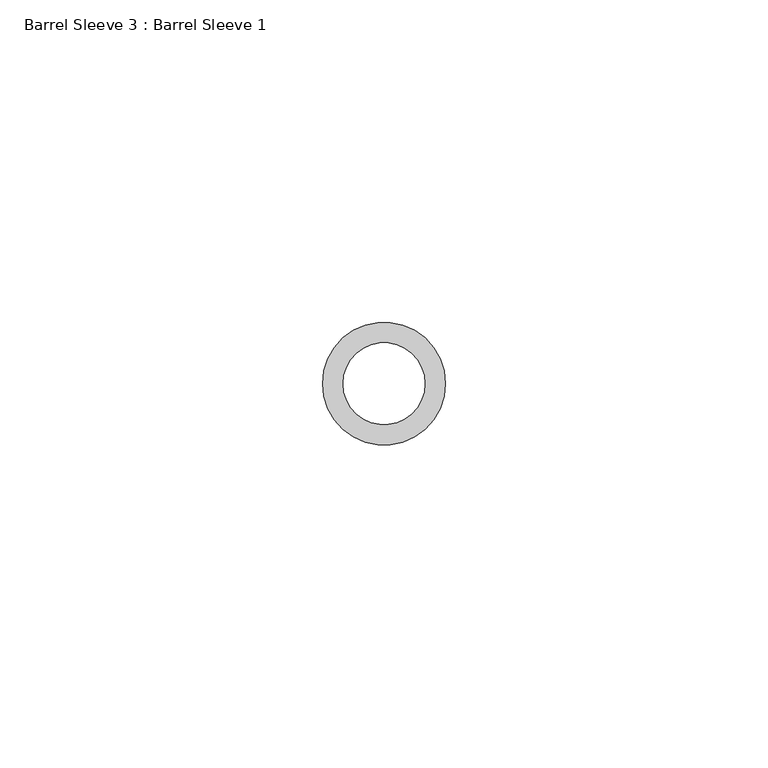
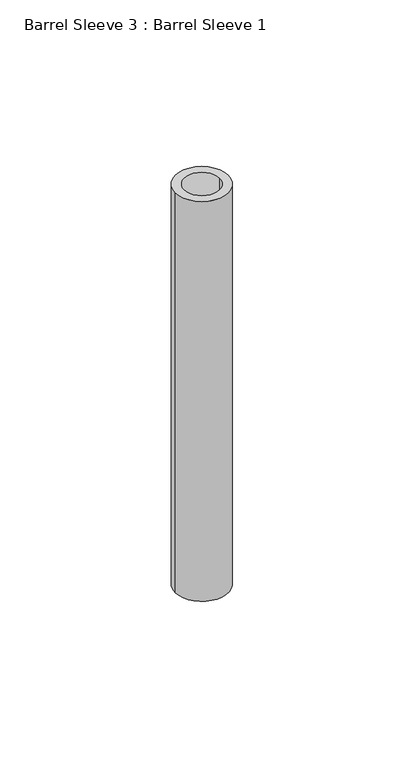
"""IFC4 building model written with IfcOpenShell, lengths in millimetres: proxy geometry, Barrel Sleeve 3 : Barrel Sleeve 1."""

from ifc_helpers import new_model, si_unit, point, frame, frame_2d, origin, place, context, project, spatial, circle_curve, trimmed, segment, composite_curve, outline, extrude, source, transform, mapped, element, save


def barrel_sleeve_3_barrel_sleeve_1_ca58ef70(model_context):
    return source(origin(), model_context, "Body", "SweptSolid", [
        extrude(outline(composite_curve([segment(trimmed(circle_curve(frame_2d((587309.5435739, -532839.3663841)), 9.525), [point((587300.0185739, -532839.3663841))], [point((587319.068574, -532839.3663841))], False, "CARTESIAN"), True, "CONTINUOUS"), segment(trimmed(circle_curve(frame_2d((587309.5435739, -532839.3663841)), 9.525), [point((587319.068574, -532839.3663841))], [point((587300.0185739, -532839.3663841))], False, "CARTESIAN"), True, "CONTINUOUS")], self_intersect=False), holes=[composite_curve([segment(trimmed(circle_curve(frame_2d((587309.5435739, -532839.3663841)), 6.35), [point((587303.1935739, -532839.3663841))], [point((587315.893574, -532839.3663841))], True, "CARTESIAN"), True, "CONTINUOUS"), segment(trimmed(circle_curve(frame_2d((587309.5435739, -532839.3663841)), 6.35), [point((587315.893574, -532839.3663841))], [point((587303.1935739, -532839.3663841))], True, "CARTESIAN"), True, "CONTINUOUS")], self_intersect=False)]), frame((0.0, 0.0, -152.4), z_axis=(0.0, 0.0, 1.0), x_axis=(1.0, 0.0, 0.0)), (0.0, 0.0, 1.0), 152.4),
    ])


if __name__ == "__main__":
    model = new_model("IFC4")
    model_context = context("Model", 3, world=origin())
    ifc_project = project(units=[si_unit("LENGTHUNIT", "METRE", prefix="MILLI")], contexts=[model_context])
    site = spatial("IfcSite", under=ifc_project)
    building = spatial("IfcBuilding", under=site)
    placement = place(None, origin())
    barrel_sleeve_3_barrel_sleeve_1_shape = barrel_sleeve_3_barrel_sleeve_1_ca58ef70(model_context)
    element("IfcBuildingElementProxy", 1, Name="Barrel Sleeve 3 : Barrel Sleeve 1", ObjectType="Barrel Sleeve 3 : Barrel Sleeve 1", at=placement, inside=building, context=model_context, shape_type="MappedRepresentation", body=[
        mapped(barrel_sleeve_3_barrel_sleeve_1_shape, transform((0.0, 0.0, 0.0), x_axis=(1.0, 0.0, 0.0), y_axis=(0.0, 1.0, 0.0), z_axis=(0.0, 0.0, 1.0))),
    ])
    save(model, "model.ifc")

# Revit data of these elements
# Element 1 (IfcBuildingElementProxy, "Barrel Sleeve 3 : Barrel Sleeve 1")
#   Materials on its faces: "5/8\" ID STEEL SLEEVE"
# Materials
#   "5/8\" ID STEEL SLEEVE": class "Metal", colour RGB 189 187 185, transparency 0, Description = "Carbon steel", Cost = 0
